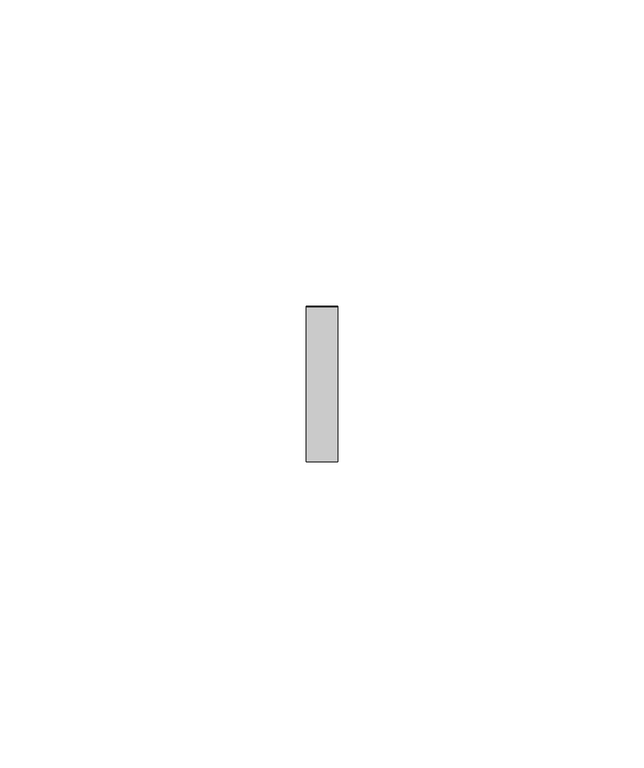
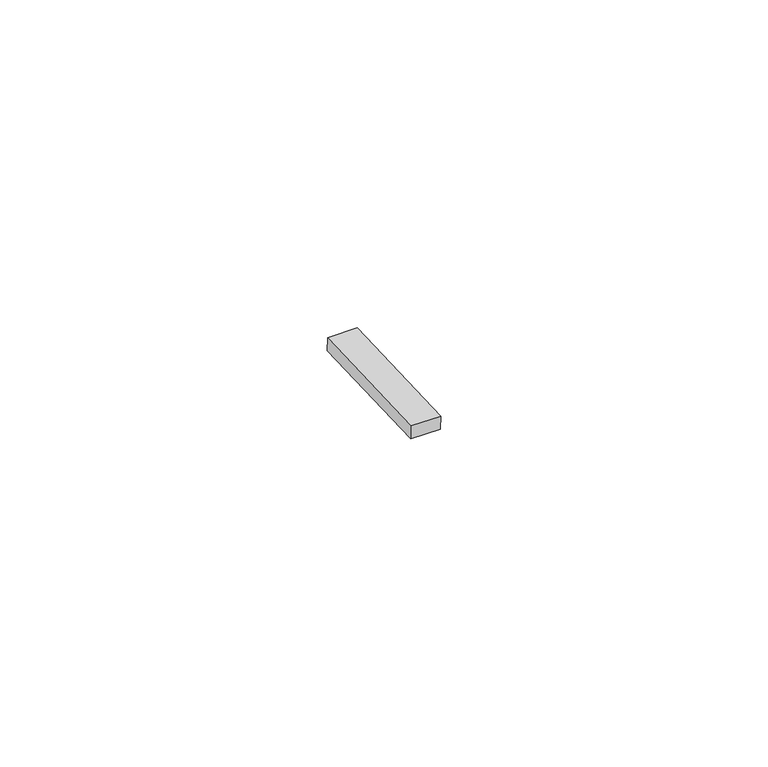
"""IFC4 building model written with IfcOpenShell, lengths in millimetres: proxy geometry, Inner panel:Inner panel:1:Inner panel:1 : Inner panel:Inner panel:300324:2:Inner panel:1:Inner panel:1 : Inner panel:Inner panel:300324:2 : Inner panel:Inner panel:1:Inner panel:1 : Inner panel:Inner panel:300324:300043:133 : Inner panel:Inner panel:1:Inner panel:1 : Inner panel:Inner panel:300324:2:Inner panel:1:Inner panel:1 : Inner panel:Inner panel:300324:2 : Inner panel:Inner panel:1:Inner panel:1 : Inner panel:Inner panel:300324:300043:308120."""

from ifc_helpers import new_model, si_unit, frame, origin, place, context, project, spatial, polyline, outline, extrude, source, transform, mapped, element, save


def generic_models_57bdcac5(model_context):
    return source(origin(), model_context, "Body", "SweptSolid", [
        extrude(outline(polyline([(0.0, -25.4), (0.0, 0.0), (5.2138089, 0.0), (5.2138089, -25.4), (0.0, -25.4)])), frame((591904.595117, -576574.3073926, 4050.9976844), z_axis=(0.0, -0.041630544712223896, 0.9991330730923502), x_axis=(-1.0, 0.0, 0.0)), (0.0, 0.0, 1.0), 2.4763745),
    ])


if __name__ == "__main__":
    model = new_model("IFC4")
    model_context = context("Model", 3, world=origin())
    ifc_project = project(units=[si_unit("LENGTHUNIT", "METRE", prefix="MILLI")], contexts=[model_context])
    site = spatial("IfcSite", under=ifc_project)
    building = spatial("IfcBuilding", under=site)
    placement = place(None, origin())
    generic_models_shape = generic_models_57bdcac5(model_context)
    element("IfcBuildingElementProxy", 1, Name="Inner panel:Inner panel:1:Inner panel:1 : Inner panel:Inner panel:300324:2:Inner panel:1:Inner panel:1 : Inner panel:Inner panel:300324:2 : Inner panel:Inner panel:1:Inner panel:1 : Inner panel:Inner panel:300324:300043:133 : Inner panel:Inner panel:1:Inner panel:1 : Inner panel:Inner panel:300324:2:Inner panel:1:Inner panel:1 : Inner panel:Inner panel:300324:2 : Inner panel:Inner panel:1:Inner panel:1 : Inner panel:Inner panel:300324:300043:308120", ObjectType="Inner panel:Inner panel:1:Inner panel:1 : Inner panel:Inner panel:300324:2:Inner panel:1:Inner panel:1 : Inner panel:Inner panel:300324:2 : Inner panel:Inner panel:1:Inner panel:1 : Inner panel:Inner panel:300324:300043:133 : Inner panel:Inner panel:1:Inner panel:1 : Inner panel:Inner panel:300324:2:Inner panel:1:Inner panel:1 : Inner panel:Inner panel:300324:2 : Inner panel:Inner panel:1:Inner panel:1 : Inner panel:Inner panel:300324:300043:308120", at=placement, inside=building, context=model_context, shape_type="MappedRepresentation", body=[
        mapped(generic_models_shape, transform((0.0, 0.0, 0.0), x_axis=(1.0, 0.0, 0.0), y_axis=(0.0, 1.0, 0.0), z_axis=(0.0, 0.0, 1.0))),
    ])
    save(model, "model.ifc")

# Revit data of these elements
# Type "Inner panel:Inner panel:1:Inner panel:1 : Inner panel:Inner panel:300324:2:Inner panel:1:Inner panel:1 : Inner panel:Inner panel:300324:2 : Inner panel:Inner panel:1:Inner panel:1 : Inner panel:Inner panel:300324:300043:133 : Inner panel:Inner panel:1:Inner panel:1 : Inner panel:Inner panel:300324:2:Inner panel:1:Inner panel:1 : Inner panel:Inner panel:300324:2 : Inner panel:Inner panel:1:Inner panel:1 : Inner panel:Inner panel:300324:300043:308120"
#   NameOverride = "Inner panel:Inner panel:1:Inner panel:1 : Inner panel:Inner panel:300324:2:Inner panel:1:Inner panel:1 : Inner panel:Inner panel:300324:2 : Inner panel:Inner panel:1:Inner panel:1 : Inner panel:Inner panel:300324:300043:308120"
#   ObjectTypeOverride = "Inner panel:1:Inner panel:1 : Inner panel:Inner panel:300324:2 : Inner panel:Inner panel:1:Inner panel:1 : Inner panel:Inner panel:300324:300043"
#   Reference = "Inner panel"
#   Tag = "308120"
# Element 1 (IfcBuildingElementProxy, "Inner panel:Inner panel:1:Inner panel:1 : Inner panel:Inner panel:300324:2:Inner panel:1:Inner panel:1 : Inner panel:Inner panel:300324:2 : Inner panel:Inner panel:1:Inner panel:1 : Inner panel:Inner panel:300324:300043:133 : Inner panel:Inner panel:1:Inner panel:1 : Inner panel:Inner panel:300324:2:Inner panel:1:Inner panel:1 : Inner panel:Inner panel:300324:2 : Inner panel:Inner panel:1:Inner panel:1 : Inner panel:Inner panel:300324:300043:308120")
#   Materials on its faces: "AT CLIP - 1\" WIDE NON ABSORBENT, WEATHER-RESISTANT NEOPRENE/EPDM/SBR FOAM"
# Materials
#   "AT CLIP - 1\" WIDE NON ABSORBENT, WEATHER-RESISTANT NEOPRENE/EPDM/SBR FOAM": class "Generic", colour RGB 85 85 85, transparency 0, Cost = 0
